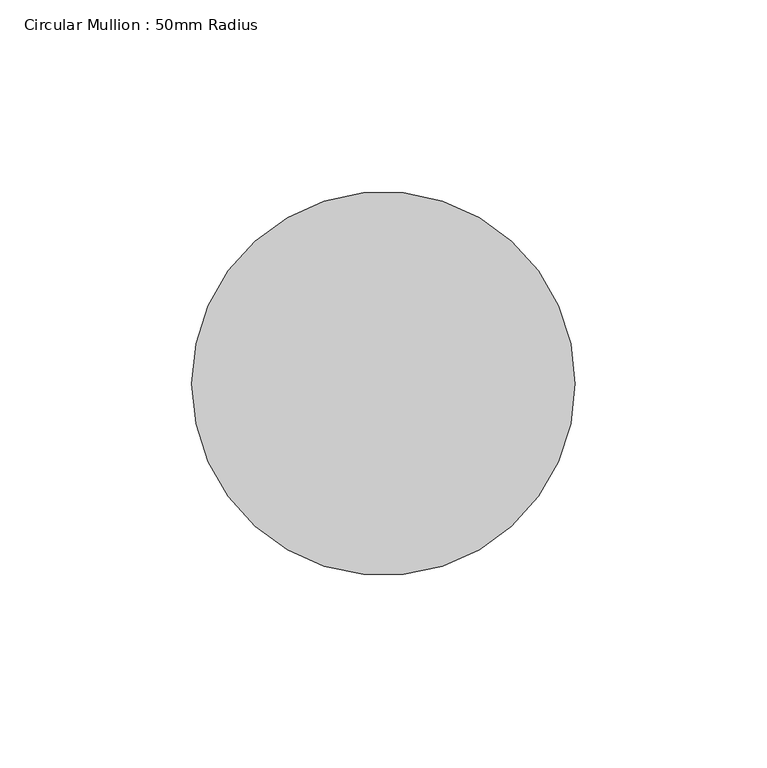
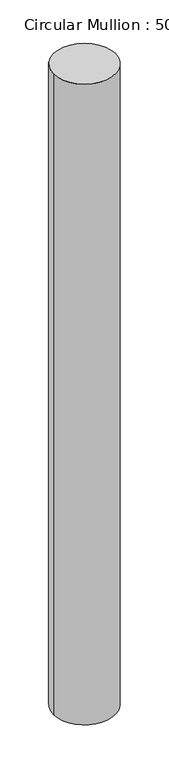
"""IFC4 building model written with IfcOpenShell, lengths in millimetres: member geometry, Circular Mullion : 50mm Radius."""

from ifc_helpers import new_model, si_unit, point, frame, origin, origin_2d, place, context, project, spatial, circle_curve, trimmed, segment, composite_curve, outline, extrude, source, transform, mapped, element, save


def circular_mullion_50mm_radius_7eea7c93(model_context):
    return source(origin(), model_context, "Body", "SweptSolid", [
        extrude(outline(composite_curve([segment(trimmed(circle_curve(origin_2d(), 50.0), [point((50.0, 0.0))], [point((-50.0, 0.0))], False, "CARTESIAN"), True, "CONTINUOUS"), segment(trimmed(circle_curve(origin_2d(), 50.0), [point((-50.0, 0.0))], [point((50.0, 0.0))], False, "CARTESIAN"), True, "CONTINUOUS")], self_intersect=False)), frame((0.0, 0.0, -1093.7811268), z_axis=(0.0, 0.0, 1.0), x_axis=(1.0, 0.0, 0.0)), (0.0, 0.0, 1.0), 1093.7811268),
    ])


if __name__ == "__main__":
    model = new_model("IFC4")
    model_context = context("Model", 3, world=origin())
    ifc_project = project(units=[si_unit("LENGTHUNIT", "METRE", prefix="MILLI")], contexts=[model_context])
    site = spatial("IfcSite", under=ifc_project)
    building = spatial("IfcBuilding", under=site)
    placement = place(None, origin())
    circular_mullion_50mm_radius_shape = circular_mullion_50mm_radius_7eea7c93(model_context)
    element("IfcMember", 1, ObjectType="Circular Mullion : 50mm Radius", at=placement, inside=building, context=model_context, shape_type="MappedRepresentation", body=[
        mapped(circular_mullion_50mm_radius_shape, transform((0.0, 0.0, 0.0), x_axis=(1.0, 0.0, 0.0), y_axis=(0.0, 1.0, 0.0), z_axis=(0.0, 0.0, 1.0))),
    ])
    save(model, "model.ifc")

# Revit data of these elements
# Type "Circular Mullion : 50mm Radius"
#   built-in parameter 1007350 = 0.164042 (stored number, unit not read)
# Element 1 (IfcMember, "Circular Mullion : 50mm Radius")
#   Materials on its faces: "Aluminium"
# Materials
#   "Aluminium": class "Metal", colour RGB 247 247 247, transparency 0, Description = "Aluminium 6061", Cost = 0
